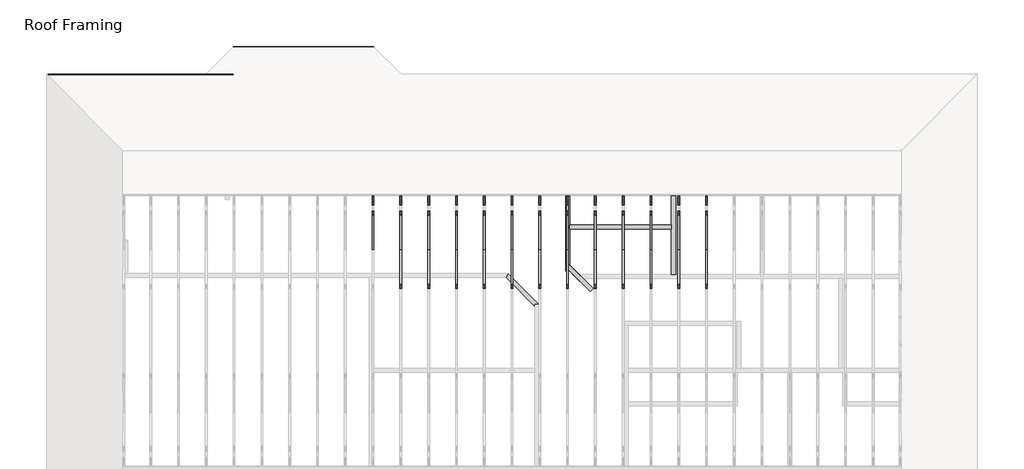
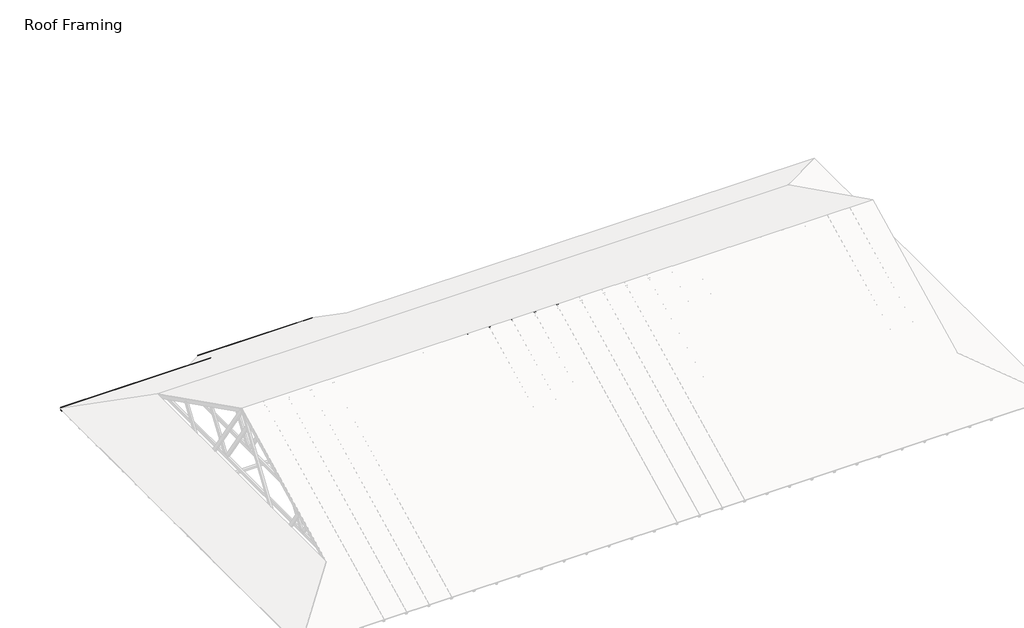
# One storey, part 6 of 7: 43 beams, 25 members.
"""IFC4 building model written with IfcOpenShell, lengths in millimetres."""

import ifcopenshell
import ifcopenshell.guid

model = None  # the IFC model being written
_history = None  # IfcOwnerHistory: only IFC2X3 demands one
_inside = {}  # id of a spatial element -> (the spatial element, [elements in it])
_under = {}  # id of a project, library or spatial element -> (it, [spatial elements below it])
_declared = {}  # id of a project -> (the project, [libraries it declares])
_typed = {}  # id of a type object -> (the type object, [elements of that type])
_made_of = {}  # id of a material, layer set ... -> (it, [elements and type objects made of it])


def new_model(schema):
    """Start an empty IFC model of exactly this schema.

    Asked for "IFC4X3", IfcOpenShell would pick the latest addendum, in which some entities
    have other attributes; the version numbers below select the first issue.
    IFC2X3 requires an IfcOwnerHistory on every rooted entity: one is made here for all.
    """
    global model, _history
    if schema == "IFC4X3":
        model = ifcopenshell.file(schema_version=(4, 3, 0, 0))
    else:
        model = ifcopenshell.file(schema=schema)
    _inside.clear()
    _under.clear()
    _declared.clear()
    _typed.clear()
    _made_of.clear()
    _history = None
    if model.schema == "IFC2X3":
        org = make("IfcOrganization", Name="unknown")
        user = make(
            "IfcPersonAndOrganization",
            ThePerson=make("IfcPerson", FamilyName="unknown"),
            TheOrganization=org,
        )
        app = make(
            "IfcApplication",
            ApplicationDeveloper=org,
            Version="unknown",
            ApplicationFullName="unknown",
            ApplicationIdentifier="unknown",
        )
        _history = make(
            "IfcOwnerHistory",
            OwningUser=user,
            OwningApplication=app,
            ChangeAction="ADDED",
            CreationDate=0,
        )
    return model


def make(cls, **values):
    """One entity of the class cls with the attributes given. An attribute that is None is left unset."""
    return model.create_entity(
        cls, **{name: value for name, value in values.items() if value is not None}
    )


def rooted(cls, **values):
    """An entity with a GlobalId (a new one), such as an element, a storey or a relation."""
    return make(cls, GlobalId=ifcopenshell.guid.new(), OwnerHistory=_history, **values)


def si_unit(unit_type, name, prefix=None):
    """IfcSIUnit, for example si_unit("LENGTHUNIT", "METRE", prefix="MILLI")."""
    return make("IfcSIUnit", UnitType=unit_type, Prefix=prefix, Name=name)


def assignment(units):
    """IfcUnitAssignment: the units of a project."""
    return None if units is None else make("IfcUnitAssignment", Units=units)


def point(xyz):
    """IfcCartesianPoint."""
    return None if xyz is None else make("IfcCartesianPoint", Coordinates=xyz)


def direction(xyz):
    """IfcDirection."""
    return None if xyz is None else make("IfcDirection", DirectionRatios=xyz)


def frame(location, z_axis=None, x_axis=None):
    """IfcAxis2Placement3D, a coordinate frame: its origin and axes. An axis left out is left unset."""
    return make(
        "IfcAxis2Placement3D",
        Location=point(location),
        Axis=direction(z_axis),
        RefDirection=direction(x_axis),
    )


def origin():
    """The frame at (0, 0, 0) with its axes left unset."""
    return frame((0.0, 0.0, 0.0))


def place(relative_to, where):
    """IfcLocalPlacement: puts the frame where relative to a parent placement (None: the world)."""
    return make(
        "IfcLocalPlacement", PlacementRelTo=relative_to, RelativePlacement=where
    )


def context(
    kind, dimensions, precision=None, world=None, true_north=None, identifier=None
):
    """IfcGeometricRepresentationContext, for example the 3D "Model" context."""
    return make(
        "IfcGeometricRepresentationContext",
        ContextIdentifier=identifier,
        ContextType=kind,
        CoordinateSpaceDimension=dimensions,
        Precision=precision,
        WorldCoordinateSystem=world,
        TrueNorth=true_north,
    )


def project(units=None, contexts=None):
    """IfcProject with its units and contexts."""
    return rooted(
        "IfcProject",
        Name="project",
        RepresentationContexts=contexts,
        UnitsInContext=assignment(units),
    )


def spatial(cls, under=None, at=None, **own):
    """A site, building, storey or space (cls), placed at a placement, below another one or the project."""
    s = rooted(cls, ObjectPlacement=at, **own)
    if under is not None:
        _under.setdefault(under.id(), (under, []))[1].append(s)
    return s


def polyline(points):
    """IfcPolyline through the points."""
    return make("IfcPolyline", Points=[point(p) for p in points])


def outline(outer, holes=None, kind="AREA"):
    """IfcArbitraryClosedProfileDef: a profile drawn as a closed curve; with holes, ...WithVoids."""
    if holes is None:
        return make("IfcArbitraryClosedProfileDef", ProfileType=kind, OuterCurve=outer)
    return make(
        "IfcArbitraryProfileDefWithVoids",
        ProfileType=kind,
        OuterCurve=outer,
        InnerCurves=holes,
    )


def extrude(swept, where, along, depth):
    """IfcExtrudedAreaSolid: the profile swept, set in the frame where, extruded along a direction by depth."""
    return make(
        "IfcExtrudedAreaSolid",
        SweptArea=swept,
        Position=where,
        ExtrudedDirection=direction(along),
        Depth=depth,
    )


def faces_of(points, faces, orient=None, outer=None):
    """IfcFace entities. A face is a list of loops; a loop is a list of indices into points, from 0.

    orient and outer hold one flag for each loop. By default every Orientation is true, the
    first loop of a face is its IfcFaceOuterBound and the others are IfcFaceBound.
    """
    made = []
    for i, loops in enumerate(faces):
        bounds = []
        for j, loop in enumerate(loops):
            is_outer = j == 0 if outer is None else outer[i][j]
            bounds.append(
                make(
                    "IfcFaceOuterBound" if is_outer else "IfcFaceBound",
                    Bound=make("IfcPolyLoop", Polygon=[points[k] for k in loop]),
                    Orientation=True if orient is None else orient[i][j],
                )
            )
        made.append(make("IfcFace", Bounds=bounds))
    return made


def faceted_brep(points, faces, orient=None, outer=None, voids=None):
    """IfcFacetedBrep: a solid bounded by flat faces; with voids (closed shells), ...WithVoids."""
    shared = [point(p) for p in points]
    hull = make("IfcClosedShell", CfsFaces=faces_of(shared, faces, orient, outer))
    if voids is None:
        return make("IfcFacetedBrep", Outer=hull)
    return make(
        "IfcFacetedBrepWithVoids",
        Outer=hull,
        Voids=[
            make(cls, CfsFaces=faces_of(shared, fs, o, b)) for cls, fs, o, b in voids
        ],
    )


def shape(context_of_items, identifier, shape_type, items):
    """IfcShapeRepresentation: the items that make up one representation, for example the "Body"."""
    return make(
        "IfcShapeRepresentation",
        ContextOfItems=context_of_items,
        RepresentationIdentifier=identifier,
        RepresentationType=shape_type,
        Items=items,
    )


def source(mapping_origin, context_of_items, identifier, shape_type, items):
    """IfcRepresentationMap: a shape defined once, which mapped items show again and again."""
    return make(
        "IfcRepresentationMap",
        MappingOrigin=mapping_origin,
        MappedRepresentation=shape(context_of_items, identifier, shape_type, items),
    )


def transform(
    local_origin,
    x_axis=None,
    y_axis=None,
    z_axis=None,
    scale=None,
    scale2=None,
    scale3=None,
    uniform=True,
):
    """IfcCartesianTransformationOperator3D, or its non-uniform kind. x_axis, y_axis, z_axis: its Axis1, 2, 3."""
    if uniform:
        return make(
            "IfcCartesianTransformationOperator3D",
            Axis1=direction(x_axis),
            Axis2=direction(y_axis),
            LocalOrigin=point(local_origin),
            Scale=scale,
            Axis3=direction(z_axis),
        )
    return make(
        "IfcCartesianTransformationOperator3DnonUniform",
        Axis1=direction(x_axis),
        Axis2=direction(y_axis),
        LocalOrigin=point(local_origin),
        Scale=scale,
        Axis3=direction(z_axis),
        Scale2=scale2,
        Scale3=scale3,
    )


def mapped(mapping_source, mapping_target):
    """IfcMappedItem: shows the shape of a source again, moved by a transform."""
    return make(
        "IfcMappedItem", MappingSource=mapping_source, MappingTarget=mapping_target
    )


def made_of(thing, what):
    """Note that an element or type object is made of a material, layer set ...; save() writes the relation."""
    if what is not None:
        _made_of.setdefault(what.id(), (what, []))[1].append(thing)
    return thing


def element(
    cls,
    number,
    at=None,
    inside=None,
    cuts=None,
    type_object=None,
    material=None,
    context=None,
    identifier="Body",
    shape_type=None,
    held_by="IfcProductDefinitionShape",
    body=None,
    shapes=None,
    **own,
):
    """One element of the class cls, such as IfcWall. Its Tag is "e" and its number.

    at: its placement. inside: the storey or other place that contains it. cuts: it is an
    opening in that element (IfcRelVoidsElement). A single representation is given by context,
    identifier, shape_type and body (its items); several are given by shapes. held_by: the class
    of the entity that holds the representations. save() writes the other relations.
    """
    e = rooted(cls, Tag="e%d" % number, ObjectPlacement=at, **own)
    if body is not None:
        shapes = [shape(context, identifier, shape_type, body)]
    if shapes is not None:
        e.Representation = make(held_by, Representations=shapes)
    if inside is not None:
        _inside.setdefault(inside.id(), (inside, []))[1].append(e)
    if cuts is not None:
        rooted(
            "IfcRelVoidsElement", RelatingBuildingElement=cuts, RelatedOpeningElement=e
        )
    if type_object is not None:
        _typed.setdefault(type_object.id(), (type_object, []))[1].append(e)
    return made_of(e, material)


def aggregate(whole, parts):
    """IfcRelAggregates: a whole, such as a stair, and the parts it consists of."""
    return rooted("IfcRelAggregates", RelatingObject=whole, RelatedObjects=parts)


def save(model, path):
    """Write the relations noted so far, then the file.

    IfcRelAggregates (storeys below a building ...), IfcRelContainedInSpatialStructure (elements
    in a storey), IfcRelDefinesByType, IfcRelAssociatesMaterial and IfcRelDeclares: one each for
    every whole, place, type object, material and project.
    """
    for whole, parts in _under.values():
        aggregate(whole, parts)
    for where, things in _inside.values():
        rooted(
            "IfcRelContainedInSpatialStructure",
            RelatedElements=things,
            RelatingStructure=where,
        )
    for kind, things in _typed.values():
        rooted("IfcRelDefinesByType", RelatedObjects=things, RelatingType=kind)
    for what, things in _made_of.values():
        rooted("IfcRelAssociatesMaterial", RelatedObjects=things, RelatingMaterial=what)
    for by, libraries in _declared.values():
        rooted("IfcRelDeclares", RelatingContext=by, RelatedDefinitions=libraries)
    model.write(path)


def dimension_lumber_bf031064(model_context):
    return source(origin(), model_context, "Body", "SweptSolid", [
        extrude(outline(polyline([(13801.725, 19.05), (13801.725, -19.05), (-5743.575, -19.05), (-5743.575, 19.05), (13801.725, 19.05)])), frame((0.0, 0.0, -44.45), z_axis=(0.0, 0.0, 1.0), x_axis=(1.0, 0.0, 0.0)), (0.0, 0.0, 1.0), 88.9),
    ])


def dimension_lumber_94c0e0a3(model_context):
    return source(origin(), model_context, "Body", "SweptSolid", [
        extrude(outline(polyline([(1162.05, 44.45), (1162.05, -44.45), (-1073.15, -44.45), (-1073.15, 44.45), (1162.05, 44.45)])), frame((0.0, 0.0, -19.05), z_axis=(0.0, 0.0, 1.0), x_axis=(1.0, 0.0, 0.0)), (0.0, 0.0, 1.0), 38.1),
    ])


def dimension_lumber_901b61d8(model_context):
    return source(origin(), model_context, "Body", "SweptSolid", [
        extrude(outline(polyline([(1117.6, 44.45), (1117.6, -44.45), (-1117.6, -44.45), (-1117.6, 44.45), (1117.6, 44.45)])), frame((0.0, 0.0, -19.05), z_axis=(0.0, 0.0, 1.0), x_axis=(1.0, 0.0, 0.0)), (0.0, 0.0, 1.0), 38.1),
    ])


def dimension_lumber_386be09e(model_context):
    return source(origin(), model_context, "Body", "SweptSolid", [
        extrude(outline(polyline([(1073.15, 44.45), (1073.15, -44.45), (-1073.15, -44.45), (-1073.15, 44.45), (1073.15, 44.45)])), frame((0.0, 0.0, -19.05), z_axis=(0.0, 0.0, 1.0), x_axis=(1.0, 0.0, 0.0)), (0.0, 0.0, 1.0), 38.1),
    ])


def dimension_lumber_2a703131(model_context):
    return source(origin(), model_context, "Body", "SweptSolid", [
        extrude(outline(polyline([(6275.3875, 44.45), (6275.3875, -44.45), (-6338.8875, -44.45), (-6338.8875, 44.45), (6275.3875, 44.45)])), frame((0.0, 0.0, -19.05), z_axis=(0.0, 0.0, 1.0), x_axis=(1.0, 0.0, 0.0)), (0.0, 0.0, 1.0), 38.1),
    ])


model = new_model("IFC4")

# Units and contexts
model_context = context("Model", 3, world=origin())
ifc_project = project(units=[si_unit("LENGTHUNIT", "METRE", prefix="MILLI")], contexts=[model_context])

# Site, building, storey
site = spatial("IfcSite", under=ifc_project)
building = spatial("IfcBuilding", under=site)
storey = spatial("IfcBuildingStorey", under=building, Name="Roof Framing", Elevation=2768.6)

# Beams
placement = place(None, origin())
element("IfcBeam", 1, ObjectType="Dimension Lumber : Top Supporting Lumbers", at=placement, inside=storey, context=model_context, shape_type="SweptSolid", body=[
    extrude(outline(polyline([(466.1639833, 4361.0431112), (-207.4454144, 5034.6525089), (-144.5836215, 5097.5143017), (529.0257761, 4423.904904), (466.1639833, 4361.0431112)])), frame((0.0, 0.0, 2425.7), z_axis=(0.0, 0.0, 1.0), x_axis=(1.0, 0.0, 0.0)), (0.0, 0.0, 1.0), 38.1),
    extrude(outline(polyline([(466.1639833, 4361.0431112), (-181.7263108, 5008.9334053), (-145.3540057, 5096.7439175), (-144.5836215, 5097.5143017), (529.0257761, 4423.904904), (466.1639833, 4361.0431112)])), frame((0.0, 0.0, 2425.7), z_axis=(0.0, 0.0, 1.0), x_axis=(1.0, 0.0, 0.0)), (0.0, 0.0, 1.0), 38.1),
    extrude(outline(polyline([(427.8736892, 4399.3334053), (-181.7263108, 5008.9334053), (-145.3540057, 5096.7439175), (-144.5836215, 5097.5143017), (529.0257761, 4423.904904), (504.4542774, 4399.3334053), (427.8736892, 4399.3334053)])), frame((0.0, 0.0, 2425.7), z_axis=(0.0, 0.0, 1.0), x_axis=(1.0, 0.0, 0.0)), (0.0, 0.0, 1.0), 38.1),
    extrude(outline(polyline([(427.8736892, 4399.3334053), (-181.7263108, 5008.9334053), (-145.3540057, 5096.7439175), (-144.5836215, 5097.5143017), (472.6347749, 4480.2959053), (472.6347749, 4399.3334053), (427.8736892, 4399.3334053)])), frame((0.0, 0.0, 2425.7), z_axis=(0.0, 0.0, 1.0), x_axis=(1.0, 0.0, 0.0)), (0.0, 0.0, 1.0), 38.1),
    extrude(outline(polyline([(427.8736892, 4399.3334053), (-181.7263108, 5008.9334053), (-145.3540057, 5096.7439175), (-144.5836215, 5097.5143017), (464.6972749, 4488.2334053), (464.6972749, 4399.3334053), (427.8736892, 4399.3334053)])), frame((0.0, 0.0, 2425.7), z_axis=(0.0, 0.0, 1.0), x_axis=(1.0, 0.0, 0.0)), (0.0, 0.0, 1.0), 38.1),
])
element("IfcBeam", 2, ObjectType="Dimension Lumber : Top Supporting Lumbers", at=placement, inside=storey, context=model_context, shape_type="SweptSolid", body=[
    extrude(outline(polyline([(-149.1478744, 5102.0785546), (529.0257761, 4423.904904), (466.1639833, 4361.0431112), (-212.0096673, 5039.2167618), (-149.1478744, 5102.0785546)])), frame((0.0, 0.0, 2387.6), z_axis=(0.0, 0.0, 1.0), x_axis=(1.0, 0.0, 0.0)), (0.0, 0.0, 1.0), 38.1),
    extrude(outline(polyline([(-144.9027251, 5097.8334053), (529.0257761, 4423.904904), (466.1639833, 4361.0431112), (-181.7263108, 5008.9334053), (-144.9027251, 5097.8334053)])), frame((0.0, 0.0, 2387.6), z_axis=(0.0, 0.0, 1.0), x_axis=(1.0, 0.0, 0.0)), (0.0, 0.0, 1.0), 38.1),
    extrude(outline(polyline([(-144.9027251, 5097.8334053), (529.0257761, 4423.904904), (504.4542774, 4399.3334053), (427.8736892, 4399.3334053), (-181.7263108, 5008.9334053), (-144.9027251, 5097.8334053)])), frame((0.0, 0.0, 2387.6), z_axis=(0.0, 0.0, 1.0), x_axis=(1.0, 0.0, 0.0)), (0.0, 0.0, 1.0), 38.1),
    extrude(outline(polyline([(-144.9027251, 5097.8334053), (472.6347749, 4480.2959053), (472.6347749, 4399.3334053), (427.8736892, 4399.3334053), (-181.7263108, 5008.9334053), (-144.9027251, 5097.8334053)])), frame((0.0, 0.0, 2387.6), z_axis=(0.0, 0.0, 1.0), x_axis=(1.0, 0.0, 0.0)), (0.0, 0.0, 1.0), 38.1),
    extrude(outline(polyline([(-144.9027251, 5097.8334053), (464.6972749, 4488.2334053), (464.6972749, 4399.3334053), (427.8736892, 4399.3334053), (-181.7263108, 5008.9334053), (-144.9027251, 5097.8334053)])), frame((0.0, 0.0, 2387.6), z_axis=(0.0, 0.0, 1.0), x_axis=(1.0, 0.0, 0.0)), (0.0, 0.0, 1.0), 38.1),
])
element("IfcBeam", 3, ObjectType="Dimension Lumber : Roof Lumbers", at=placement, inside=storey, context=model_context, shape_type="Brep", body=[
    faceted_brep([(-6671.1152251, 4918.4459053, 2653.50625), (-6671.1152251, 4956.5459053, 2653.50625), (-6671.1152251, 4956.5459053, 2564.60625), (-6671.1152251, 4918.4459053, 2564.60625), (-2613.4652251, 4918.4459053, 2653.50625), (-2613.4652251, 4918.4459053, 2564.60625), (-2613.4652251, 4956.5459053, 2564.60625), (-2613.4652251, 4956.5459053, 2653.50625)], [[[0, 1, 2, 3]], [[4, 5, 6, 7]], [[1, 0, 4, 7]], [[2, 1, 7, 6]], [[3, 2, 6, 5]], [[0, 3, 5, 4]]]),
    faceted_brep([(-6671.1152251, 4956.5459053, 2634.3548743), (-6671.1152251, 4956.5459053, 2564.60625), (-6671.1152251, 4918.4459053, 2564.60625), (-6671.1152251, 4918.4459053, 2653.50625), (-2613.4652251, 4956.5459053, 2634.3548743), (-2613.4652251, 4956.5459053, 2564.60625), (-2613.4652251, 4918.4459053, 2564.60625), (-2613.4652251, 4918.4459053, 2653.50625)], [[[0, 1, 2, 3]], [[1, 0, 4, 5]], [[2, 1, 5, 6]], [[3, 2, 6, 7]], [[7, 6, 5, 4]], [[0, 3, 7, 4]]]),
])
element("IfcBeam", 4, ObjectType="Dimension Lumber : Roof Lumbers", at=placement, inside=storey, context=model_context, shape_type="Brep", body=[
    faceted_brep([(-2613.4652251, 5528.0459053, 2348.70625), (-2613.4652251, 5566.1459053, 2348.70625), (-2613.4652251, 5566.1459053, 2259.80625), (-2613.4652251, 5528.0459053, 2259.80625), (472.6347749, 5528.0459053, 2348.70625), (472.6347749, 5528.0459053, 2259.80625), (472.6347749, 5566.1459053, 2259.80625), (472.6347749, 5566.1459053, 2348.70625)], [[[0, 1, 2, 3]], [[4, 5, 6, 7]], [[1, 0, 4, 7]], [[2, 1, 7, 6]], [[3, 2, 6, 5]], [[0, 3, 5, 4]]]),
    faceted_brep([(-2613.4652251, 5566.1459053, 2329.5548743), (-2613.4652251, 5566.1459053, 2259.80625), (-2613.4652251, 5528.0459053, 2259.80625), (-2613.4652251, 5528.0459053, 2348.70625), (472.6347749, 5566.1459053, 2329.5548743), (472.6347749, 5566.1459053, 2259.80625), (472.6347749, 5528.0459053, 2259.80625), (472.6347749, 5528.0459053, 2348.70625)], [[[0, 1, 2, 3]], [[1, 0, 4, 5]], [[2, 1, 5, 6]], [[3, 2, 6, 7]], [[7, 6, 5, 4]], [[0, 3, 7, 4]]]),
])
element("IfcBeam", 5, ObjectType="Dimension Lumber : Roof Lumbers", at=placement, inside=storey, context=model_context, shape_type="SweptSolid", body=[
    extrude(outline(polyline([(-2613.4652251, 5108.9459053), (-2613.4652251, 5147.0459053), (472.6347749, 5147.0459053), (472.6347749, 5108.9459053), (-2613.4652251, 5108.9459053)])), frame((0.0, 0.0, 2259.80625), z_axis=(0.0, 0.0, 1.0), x_axis=(1.0, 0.0, 0.0)), (0.0, 0.0, 1.0), 88.9),
])
element("IfcBeam", 6, ObjectType="Dimension Lumber : Top Supporting Lumbers", at=placement, inside=storey, context=model_context, shape_type="SweptSolid", body=[
    extrude(outline(polyline([(4765.2347749, 638.6232039), (4676.3347749, 638.6232039), (4676.3347749, 4399.3334053), (4765.2347749, 4399.3334053), (4765.2347749, 638.6232039)])), frame((0.0, 0.0, 2692.4), z_axis=(0.0, 0.0, 1.0), x_axis=(1.0, 0.0, 0.0)), (0.0, 0.0, 1.0), 38.1),
    extrude(outline(polyline([(4676.3347749, 727.4459053), (4676.3347749, 4399.3334053), (4765.2347749, 4399.3334053), (4765.2347749, 764.269491), (4676.3347749, 727.4459053)])), frame((0.0, 0.0, 2692.4), z_axis=(0.0, 0.0, 1.0), x_axis=(1.0, 0.0, 0.0)), (0.0, 0.0, 1.0), 38.1),
])
element("IfcBeam", 7, ObjectType="Dimension Lumber : Top Supporting Lumbers", at=placement, inside=storey, context=model_context, shape_type="SweptSolid", body=[
    extrude(outline(polyline([(5056.0583606, 473.4459053), (4993.1965677, 410.5841125), (4676.3347749, 727.4459053), (4765.2347749, 764.269491), (5056.0583606, 473.4459053)])), frame((0.0, 0.0, 2692.4), z_axis=(0.0, 0.0, 1.0), x_axis=(1.0, 0.0, 0.0)), (0.0, 0.0, 1.0), 38.1),
    extrude(outline(polyline([(4930.3347749, 473.4459053), (4676.3347749, 727.4459053), (4765.2347749, 764.269491), (4967.1583606, 562.3459053), (4930.3347749, 473.4459053)])), frame((0.0, 0.0, 2692.4), z_axis=(0.0, 0.0, 1.0), x_axis=(1.0, 0.0, 0.0)), (0.0, 0.0, 1.0), 38.1),
])
element("IfcBeam", 8, ObjectType="Dimension Lumber : Top Supporting Lumbers", at=placement, inside=storey, context=model_context, shape_type="SweptSolid", body=[
    extrude(outline(polyline([(4086.2782231, -98.5475429), (4023.4164303, -161.4093358), (3372.6861892, 489.3209053), (3409.5097749, 578.2209053), (4086.2782231, -98.5475429)])), frame((0.0, 0.0, 2692.4), z_axis=(0.0, 0.0, 1.0), x_axis=(1.0, 0.0, 0.0)), (0.0, 0.0, 1.0), 38.1),
    extrude(outline(polyline([(3996.8847749, -134.8776804), (3372.6861892, 489.3209053), (3409.5097749, 578.2209053), (4085.7847749, -98.0540947), (3996.8847749, -134.8776804)])), frame((0.0, 0.0, 2692.4), z_axis=(0.0, 0.0, 1.0), x_axis=(1.0, 0.0, 0.0)), (0.0, 0.0, 1.0), 38.1),
])
element("IfcBeam", 9, ObjectType="Dimension Lumber : Top Supporting Lumbers", at=placement, inside=storey, context=model_context, shape_type="SweptSolid", body=[
    extrude(outline(polyline([(4676.3347749, 4399.3334053), (4765.2347749, 4399.3334053), (4765.2347749, 764.269491), (4676.3347749, 727.4459053), (4676.3347749, 4399.3334053)])), frame((0.0, 0.0, 2730.5), z_axis=(0.0, 0.0, 1.0), x_axis=(1.0, 0.0, 0.0)), (0.0, 0.0, 1.0), 38.1),
])
element("IfcBeam", 10, ObjectType="Dimension Lumber : Top Supporting Lumbers", at=placement, inside=storey, context=model_context, shape_type="SweptSolid", body=[
    extrude(outline(polyline([(4677.0339804, 726.7466998), (4739.8957732, 789.6084927), (5281.6079113, 247.8963545), (5218.7461185, 185.0345617), (4677.0339804, 726.7466998)])), frame((0.0, 0.0, 2730.5), z_axis=(0.0, 0.0, 1.0), x_axis=(1.0, 0.0, 0.0)), (0.0, 0.0, 1.0), 38.1),
    extrude(outline(polyline([(4677.0339804, 726.7466998), (4678.7220117, 728.4347312), (4765.2347749, 764.269491), (5281.6079113, 247.8963545), (5218.7461185, 185.0345617), (4677.0339804, 726.7466998)])), frame((0.0, 0.0, 2730.5), z_axis=(0.0, 0.0, 1.0), x_axis=(1.0, 0.0, 0.0)), (0.0, 0.0, 1.0), 38.1),
    extrude(outline(polyline([(4677.0339804, 726.7466998), (4678.7220117, 728.4347312), (4765.2347749, 764.269491), (4967.1583606, 562.3459053), (4930.3347749, 473.4459053), (4677.0339804, 726.7466998)])), frame((0.0, 0.0, 2730.5), z_axis=(0.0, 0.0, 1.0), x_axis=(1.0, 0.0, 0.0)), (0.0, 0.0, 1.0), 38.1),
])
dimension_lumber_shape = dimension_lumber_bf031064(model_context)
element("IfcBeam", 11, ObjectType="Dimension Lumber : Roof Lumbers", at=placement, inside=storey, context=model_context, shape_type="MappedRepresentation", body=[
    mapped(dimension_lumber_shape, transform((7511.6097749, 4518.3959053, 2609.05625), x_axis=(-1.0, 0.0, 0.0), y_axis=(0.0, -1.0, 0.0), z_axis=(0.0, 0.0, 1.0))),
])
dimension_lumber_2_shape = dimension_lumber_94c0e0a3(model_context)
element("IfcBeam", 12, ObjectType="Dimension Lumber : Top Supporting Lumbers", at=placement, inside=storey, context=model_context, shape_type="MappedRepresentation", body=[
    mapped(dimension_lumber_2_shape, transform((7044.8847749, 1635.4959053, 2711.45), x_axis=(0.0, 1.0, 0.0), y_axis=(-1.0, 0.0, 0.0), z_axis=(0.0, 0.0, 1.0))),
])
dimension_lumber_3_shape = dimension_lumber_901b61d8(model_context)
element("IfcBeam", 13, ObjectType="Dimension Lumber : Top Supporting Lumbers", at=placement, inside=storey, context=model_context, shape_type="MappedRepresentation", body=[
    mapped(dimension_lumber_3_shape, transform((5882.8347749, 1597.3959053, 2711.45), x_axis=(-1.0, 0.0, 0.0), y_axis=(0.0, -1.0, 0.0), z_axis=(0.0, 0.0, 1.0))),
])
element("IfcBeam", 14, ObjectType="Dimension Lumber : Top Supporting Lumbers", at=placement, inside=storey, context=model_context, shape_type="MappedRepresentation", body=[
    mapped(dimension_lumber_3_shape, transform((5882.8347749, 1597.3959053, 2749.55), x_axis=(1.0, 0.0, 0.0), y_axis=(0.0, 1.0, 0.0), z_axis=(0.0, 0.0, 1.0))),
])
dimension_lumber_4_shape = dimension_lumber_386be09e(model_context)
element("IfcBeam", 15, ObjectType="Dimension Lumber : Top Supporting Lumbers", at=placement, inside=storey, context=model_context, shape_type="MappedRepresentation", body=[
    mapped(dimension_lumber_4_shape, transform((7044.8847749, 1635.4959053, 2749.55), x_axis=(0.0, 1.0, 0.0), y_axis=(-1.0, 0.0, 0.0), z_axis=(0.0, 0.0, 1.0))),
])
dimension_lumber_5_shape = dimension_lumber_2a703131(model_context)
element("IfcBeam", 16, ObjectType="Dimension Lumber : Top Supporting Lumbers", at=placement, inside=storey, context=model_context, shape_type="MappedRepresentation", body=[
    mapped(dimension_lumber_5_shape, transform((6879.7847749, 4443.7834053, 2749.55), x_axis=(1.0, 0.0, 0.0), y_axis=(0.0, 1.0, 0.0), z_axis=(0.0, 0.0, 1.0))),
])
element("IfcBeam", 17, ObjectType="Dimension Lumber : Top Supporting Lumbers", at=placement, inside=storey, context=model_context, shape_type="MappedRepresentation", body=[
    mapped(dimension_lumber_5_shape, transform((6879.7847749, 4443.7834053, 2711.45), x_axis=(1.0, 0.0, 0.0), y_axis=(0.0, 1.0, 0.0), z_axis=(0.0, 0.0, 1.0))),
])
element("IfcBeam", 18, ObjectType="Dimension Lumber : 2x4 Blocking", at=placement, inside=storey, context=model_context, shape_type="SweptSolid", body=[
    extrude(outline(polyline([(7787.8347749, 4918.4459053), (7787.8347749, 4537.4459053), (7749.7347749, 4537.4459053), (7749.7347749, 4918.4459053), (7787.8347749, 4918.4459053)])), frame((0.0, 0.0, 2564.60625), z_axis=(0.0, 0.0, 1.0), x_axis=(1.0, 0.0, 0.0)), (0.0, 0.0, 1.0), 88.9),
    extrude(outline(polyline([(4897.2567107, 2564.60625), (4537.4459053, 2564.60625), (4537.4459053, 2653.50625), (4719.4567107, 2653.50625), (4897.2567107, 2564.60625)])), frame((7749.7347749, 0.0, 0.0), z_axis=(1.0, 0.0, 0.0), x_axis=(0.0, 1.0, 0.0)), (0.0, 0.0, 1.0), 38.1),
])
element("IfcBeam", 19, ObjectType="Dimension Lumber : 2x4 Blocking", at=placement, inside=storey, context=model_context, shape_type="SweptSolid", body=[
    extrude(outline(polyline([(7178.2347749, 4918.4459053), (7178.2347749, 4537.4459053), (7140.1347749, 4537.4459053), (7140.1347749, 4918.4459053), (7178.2347749, 4918.4459053)])), frame((0.0, 0.0, 2564.60625), z_axis=(0.0, 0.0, 1.0), x_axis=(1.0, 0.0, 0.0)), (0.0, 0.0, 1.0), 88.9),
    extrude(outline(polyline([(4897.2567107, 2564.60625), (4537.4459053, 2564.60625), (4537.4459053, 2653.50625), (4719.4567107, 2653.50625), (4897.2567107, 2564.60625)])), frame((7140.1347749, 0.0, 0.0), z_axis=(1.0, 0.0, 0.0), x_axis=(0.0, 1.0, 0.0)), (0.0, 0.0, 1.0), 38.1),
])
element("IfcBeam", 20, ObjectType="Dimension Lumber : 2x4 Blocking", at=placement, inside=storey, context=model_context, shape_type="SweptSolid", body=[
    extrude(outline(polyline([(6568.6347749, 4918.4459053), (6568.6347749, 4537.4459053), (6530.5347749, 4537.4459053), (6530.5347749, 4918.4459053), (6568.6347749, 4918.4459053)])), frame((0.0, 0.0, 2564.60625), z_axis=(0.0, 0.0, 1.0), x_axis=(1.0, 0.0, 0.0)), (0.0, 0.0, 1.0), 88.9),
    extrude(outline(polyline([(4897.2567107, 2564.60625), (4537.4459053, 2564.60625), (4537.4459053, 2653.50625), (4719.4567107, 2653.50625), (4897.2567107, 2564.60625)])), frame((6530.5347749, 0.0, 0.0), z_axis=(1.0, 0.0, 0.0), x_axis=(0.0, 1.0, 0.0)), (0.0, 0.0, 1.0), 38.1),
])
element("IfcBeam", 21, ObjectType="Dimension Lumber : 2x4 Blocking", at=placement, inside=storey, context=model_context, shape_type="SweptSolid", body=[
    extrude(outline(polyline([(5959.0347749, 4918.4459053), (5959.0347749, 4537.4459053), (5920.9347749, 4537.4459053), (5920.9347749, 4918.4459053), (5959.0347749, 4918.4459053)])), frame((0.0, 0.0, 2564.60625), z_axis=(0.0, 0.0, 1.0), x_axis=(1.0, 0.0, 0.0)), (0.0, 0.0, 1.0), 88.9),
    extrude(outline(polyline([(4897.2567107, 2564.60625), (4537.4459053, 2564.60625), (4537.4459053, 2653.50625), (4719.4567107, 2653.50625), (4897.2567107, 2564.60625)])), frame((5920.9347749, 0.0, 0.0), z_axis=(1.0, 0.0, 0.0), x_axis=(0.0, 1.0, 0.0)), (0.0, 0.0, 1.0), 38.1),
])
element("IfcBeam", 22, ObjectType="Dimension Lumber : 2x4 Blocking", at=placement, inside=storey, context=model_context, shape_type="SweptSolid", body=[
    extrude(outline(polyline([(5349.4347749, 4918.4459053), (5349.4347749, 4537.4459053), (5311.3347749, 4537.4459053), (5311.3347749, 4918.4459053), (5349.4347749, 4918.4459053)])), frame((0.0, 0.0, 2564.60625), z_axis=(0.0, 0.0, 1.0), x_axis=(1.0, 0.0, 0.0)), (0.0, 0.0, 1.0), 88.9),
    extrude(outline(polyline([(4897.2567107, 2564.60625), (4537.4459053, 2564.60625), (4537.4459053, 2653.50625), (4719.4567107, 2653.50625), (4897.2567107, 2564.60625)])), frame((5311.3347749, 0.0, 0.0), z_axis=(1.0, 0.0, 0.0), x_axis=(0.0, 1.0, 0.0)), (0.0, 0.0, 1.0), 38.1),
])
element("IfcBeam", 23, ObjectType="Dimension Lumber : 2x4 Blocking", at=placement, inside=storey, context=model_context, shape_type="SweptSolid", body=[
    extrude(outline(polyline([(4739.8347749, 4918.4459053), (4739.8347749, 4537.4459053), (4701.7347749, 4537.4459053), (4701.7347749, 4918.4459053), (4739.8347749, 4918.4459053)])), frame((0.0, 0.0, 2564.60625), z_axis=(0.0, 0.0, 1.0), x_axis=(1.0, 0.0, 0.0)), (0.0, 0.0, 1.0), 88.9),
    extrude(outline(polyline([(4897.2567107, 2564.60625), (4537.4459053, 2564.60625), (4537.4459053, 2653.50625), (4719.4567107, 2653.50625), (4897.2567107, 2564.60625)])), frame((4701.7347749, 0.0, 0.0), z_axis=(1.0, 0.0, 0.0), x_axis=(0.0, 1.0, 0.0)), (0.0, 0.0, 1.0), 38.1),
])
element("IfcBeam", 24, ObjectType="Dimension Lumber : 2x4 Blocking", at=placement, inside=storey, context=model_context, shape_type="SweptSolid", body=[
    extrude(outline(polyline([(4130.2347749, 4918.4459053), (4130.2347749, 4537.4459053), (4092.1347749, 4537.4459053), (4092.1347749, 4918.4459053), (4130.2347749, 4918.4459053)])), frame((0.0, 0.0, 2564.60625), z_axis=(0.0, 0.0, 1.0), x_axis=(1.0, 0.0, 0.0)), (0.0, 0.0, 1.0), 88.9),
    extrude(outline(polyline([(4897.2567107, 2564.60625), (4537.4459053, 2564.60625), (4537.4459053, 2653.50625), (4719.4567107, 2653.50625), (4897.2567107, 2564.60625)])), frame((4092.1347749, 0.0, 0.0), z_axis=(1.0, 0.0, 0.0), x_axis=(0.0, 1.0, 0.0)), (0.0, 0.0, 1.0), 38.1),
])
element("IfcBeam", 25, ObjectType="Dimension Lumber : 2x4 Blocking", at=placement, inside=storey, context=model_context, shape_type="SweptSolid", body=[
    extrude(outline(polyline([(3520.6347749, 4918.4459053), (3520.6347749, 4537.4459053), (3482.5347749, 4537.4459053), (3482.5347749, 4918.4459053), (3520.6347749, 4918.4459053)])), frame((0.0, 0.0, 2564.60625), z_axis=(0.0, 0.0, 1.0), x_axis=(1.0, 0.0, 0.0)), (0.0, 0.0, 1.0), 88.9),
    extrude(outline(polyline([(4897.2567107, 2564.60625), (4537.4459053, 2564.60625), (4537.4459053, 2653.50625), (4719.4567107, 2653.50625), (4897.2567107, 2564.60625)])), frame((3482.5347749, 0.0, 0.0), z_axis=(1.0, 0.0, 0.0), x_axis=(0.0, 1.0, 0.0)), (0.0, 0.0, 1.0), 38.1),
])
element("IfcBeam", 26, ObjectType="Dimension Lumber : 2x4 Blocking", at=placement, inside=storey, context=model_context, shape_type="SweptSolid", body=[
    extrude(outline(polyline([(2911.0347749, 4918.4459053), (2911.0347749, 4537.4459053), (2872.9347749, 4537.4459053), (2872.9347749, 4918.4459053), (2911.0347749, 4918.4459053)])), frame((0.0, 0.0, 2564.60625), z_axis=(0.0, 0.0, 1.0), x_axis=(1.0, 0.0, 0.0)), (0.0, 0.0, 1.0), 88.9),
    extrude(outline(polyline([(4897.2567107, 2564.60625), (4537.4459053, 2564.60625), (4537.4459053, 2653.50625), (4719.4567107, 2653.50625), (4897.2567107, 2564.60625)])), frame((2872.9347749, 0.0, 0.0), z_axis=(1.0, 0.0, 0.0), x_axis=(0.0, 1.0, 0.0)), (0.0, 0.0, 1.0), 38.1),
])
element("IfcBeam", 27, ObjectType="Dimension Lumber : 2x4 Blocking", at=placement, inside=storey, context=model_context, shape_type="SweptSolid", body=[
    extrude(outline(polyline([(434.5347749, 5147.0459053), (434.5347749, 5528.0459053), (472.6347749, 5528.0459053), (472.6347749, 5147.0459053), (434.5347749, 5147.0459053)])), frame((0.0, 0.0, 2259.80625), z_axis=(0.0, 0.0, 1.0), x_axis=(1.0, 0.0, 0.0)), (0.0, 0.0, 1.0), 88.9),
    extrude(outline(polyline([(5147.0459053, 2348.70625), (5329.0567107, 2348.70625), (5506.8567107, 2259.80625), (5147.0459053, 2259.80625), (5147.0459053, 2348.70625)])), frame((434.5347749, 0.0, 0.0), z_axis=(1.0, 0.0, 0.0), x_axis=(0.0, 1.0, 0.0)), (0.0, 0.0, 1.0), 38.1),
])
element("IfcBeam", 28, ObjectType="Dimension Lumber : 2x4 Blocking", at=placement, inside=storey, context=model_context, shape_type="SweptSolid", body=[
    extrude(outline(polyline([(2301.4347749, 4918.4459053), (2301.4347749, 4537.4459053), (2263.3347749, 4537.4459053), (2263.3347749, 4918.4459053), (2301.4347749, 4918.4459053)])), frame((0.0, 0.0, 2564.60625), z_axis=(0.0, 0.0, 1.0), x_axis=(1.0, 0.0, 0.0)), (0.0, 0.0, 1.0), 88.9),
    extrude(outline(polyline([(4897.2567107, 2564.60625), (4537.4459053, 2564.60625), (4537.4459053, 2653.50625), (4719.4567107, 2653.50625), (4897.2567107, 2564.60625)])), frame((2263.3347749, 0.0, 0.0), z_axis=(1.0, 0.0, 0.0), x_axis=(0.0, 1.0, 0.0)), (0.0, 0.0, 1.0), 38.1),
])
element("IfcBeam", 29, ObjectType="Dimension Lumber : 2x4 Blocking", at=placement, inside=storey, context=model_context, shape_type="SweptSolid", body=[
    extrude(outline(polyline([(1653.7347749, 4537.4459053), (1653.7347749, 4918.4459053), (1691.8347749, 4918.4459053), (1691.8347749, 4537.4459053), (1653.7347749, 4537.4459053)])), frame((0.0, 0.0, 2564.60625), z_axis=(0.0, 0.0, 1.0), x_axis=(1.0, 0.0, 0.0)), (0.0, 0.0, 1.0), 88.9),
    extrude(outline(polyline([(4537.4459053, 2653.50625), (4719.4567107, 2653.50625), (4897.2567107, 2564.60625), (4537.4459053, 2564.60625), (4537.4459053, 2653.50625)])), frame((1653.7347749, 0.0, 0.0), z_axis=(1.0, 0.0, 0.0), x_axis=(0.0, 1.0, 0.0)), (0.0, 0.0, 1.0), 38.1),
])
element("IfcBeam", 30, ObjectType="Dimension Lumber : 2x4 Blocking", at=placement, inside=storey, context=model_context, shape_type="SweptSolid", body=[
    extrude(outline(polyline([(1044.1347749, 4537.4459053), (1044.1347749, 4918.4459053), (1082.2347749, 4918.4459053), (1082.2347749, 4537.4459053), (1044.1347749, 4537.4459053)])), frame((0.0, 0.0, 2564.60625), z_axis=(0.0, 0.0, 1.0), x_axis=(1.0, 0.0, 0.0)), (0.0, 0.0, 1.0), 88.9),
    extrude(outline(polyline([(4537.4459053, 2653.50625), (4719.4567107, 2653.50625), (4897.2567107, 2564.60625), (4537.4459053, 2564.60625), (4537.4459053, 2653.50625)])), frame((1044.1347749, 0.0, 0.0), z_axis=(1.0, 0.0, 0.0), x_axis=(0.0, 1.0, 0.0)), (0.0, 0.0, 1.0), 38.1),
])
element("IfcBeam", 31, ObjectType="Dimension Lumber : 2x4 Truss", at=placement, inside=storey, context=model_context, shape_type="SweptSolid", body=[
    extrude(outline(polyline([(4956.5459053, 2634.3548743), (4916.7886167, 2554.840297), (-682.2540947, 5354.3616527), (-682.2540947, 5453.7548743), (4956.5459053, 2634.3548743)])), frame((7749.7347749, 0.0, 0.0), z_axis=(1.0, 0.0, 0.0), x_axis=(0.0, 1.0, 0.0)), (0.0, 0.0, 1.0), 38.1),
])
element("IfcBeam", 32, ObjectType="Dimension Lumber : 2x4 Truss", at=placement, inside=storey, context=model_context, shape_type="SweptSolid", body=[
    extrude(outline(polyline([(4956.5459053, 2634.3548743), (4916.7886167, 2554.840297), (-682.2540947, 5354.3616527), (-682.2540947, 5453.7548743), (4956.5459053, 2634.3548743)])), frame((7140.1347749, 0.0, 0.0), z_axis=(1.0, 0.0, 0.0), x_axis=(0.0, 1.0, 0.0)), (0.0, 0.0, 1.0), 38.1),
])
element("IfcBeam", 33, ObjectType="Dimension Lumber : 2x4 Truss", at=placement, inside=storey, context=model_context, shape_type="SweptSolid", body=[
    extrude(outline(polyline([(4956.5459053, 2634.3548743), (4916.7886167, 2554.840297), (-682.2540947, 5354.3616527), (-682.2540947, 5453.7548743), (4956.5459053, 2634.3548743)])), frame((6530.5347749, 0.0, 0.0), z_axis=(1.0, 0.0, 0.0), x_axis=(0.0, 1.0, 0.0)), (0.0, 0.0, 1.0), 38.1),
])
element("IfcBeam", 34, ObjectType="Dimension Lumber : 2x4 Truss", at=placement, inside=storey, context=model_context, shape_type="SweptSolid", body=[
    extrude(outline(polyline([(4956.5459053, 2634.3548743), (4916.7886167, 2554.840297), (-682.2540947, 5354.3616527), (-682.2540947, 5453.7548743), (4956.5459053, 2634.3548743)])), frame((5920.9347749, 0.0, 0.0), z_axis=(1.0, 0.0, 0.0), x_axis=(0.0, 1.0, 0.0)), (0.0, 0.0, 1.0), 38.1),
])
element("IfcBeam", 35, ObjectType="Dimension Lumber : 2x4 Truss", at=placement, inside=storey, context=model_context, shape_type="SweptSolid", body=[
    extrude(outline(polyline([(4956.5459053, 2634.3548743), (4916.7886167, 2554.840297), (-682.2540947, 5354.3616527), (-682.2540947, 5453.7548743), (4956.5459053, 2634.3548743)])), frame((5311.3347749, 0.0, 0.0), z_axis=(1.0, 0.0, 0.0), x_axis=(0.0, 1.0, 0.0)), (0.0, 0.0, 1.0), 38.1),
])
element("IfcBeam", 36, ObjectType="Dimension Lumber : 2x4 Truss", at=placement, inside=storey, context=model_context, shape_type="SweptSolid", body=[
    extrude(outline(polyline([(4956.5459053, 2634.3548743), (4916.7886167, 2554.840297), (-682.2540947, 5354.3616527), (-682.2540947, 5453.7548743), (4956.5459053, 2634.3548743)])), frame((4701.7347749, 0.0, 0.0), z_axis=(1.0, 0.0, 0.0), x_axis=(0.0, 1.0, 0.0)), (0.0, 0.0, 1.0), 38.1),
])
element("IfcBeam", 37, ObjectType="Dimension Lumber : 2x4 Truss", at=placement, inside=storey, context=model_context, shape_type="SweptSolid", body=[
    extrude(outline(polyline([(4956.5459053, 2634.3548743), (4916.7886167, 2554.840297), (-682.2540947, 5354.3616527), (-682.2540947, 5453.7548743), (4956.5459053, 2634.3548743)])), frame((4092.1347749, 0.0, 0.0), z_axis=(1.0, 0.0, 0.0), x_axis=(0.0, 1.0, 0.0)), (0.0, 0.0, 1.0), 38.1),
])
element("IfcBeam", 38, ObjectType="Dimension Lumber : 2x4 Truss", at=placement, inside=storey, context=model_context, shape_type="SweptSolid", body=[
    extrude(outline(polyline([(4956.5459053, 2634.3548743), (4916.7886167, 2554.840297), (-682.2540947, 5354.3616527), (-682.2540947, 5453.7548743), (4956.5459053, 2634.3548743)])), frame((3482.5347749, 0.0, 0.0), z_axis=(1.0, 0.0, 0.0), x_axis=(0.0, 1.0, 0.0)), (0.0, 0.0, 1.0), 38.1),
])
element("IfcBeam", 39, ObjectType="Dimension Lumber : 2x4 Truss", at=placement, inside=storey, context=model_context, shape_type="SweptSolid", body=[
    extrude(outline(polyline([(4956.5459053, 2634.3548743), (4916.7886167, 2554.840297), (-682.2540947, 5354.3616527), (-682.2540947, 5453.7548743), (4956.5459053, 2634.3548743)])), frame((2872.9347749, 0.0, 0.0), z_axis=(1.0, 0.0, 0.0), x_axis=(0.0, 1.0, 0.0)), (0.0, 0.0, 1.0), 38.1),
])
element("IfcBeam", 40, ObjectType="Dimension Lumber : 2x4 Truss", at=placement, inside=storey, context=model_context, shape_type="SweptSolid", body=[
    extrude(outline(polyline([(4956.5459053, 2634.3548743), (4916.7886167, 2554.840297), (-682.2540947, 5354.3616527), (-682.2540947, 5453.7548743), (4956.5459053, 2634.3548743)])), frame((2263.3347749, 0.0, 0.0), z_axis=(1.0, 0.0, 0.0), x_axis=(0.0, 1.0, 0.0)), (0.0, 0.0, 1.0), 38.1),
])
element("IfcBeam", 41, ObjectType="Dimension Lumber : 2x4 Truss", at=placement, inside=storey, context=model_context, shape_type="SweptSolid", body=[
    extrude(outline(polyline([(4956.5459053, 2634.3548743), (4916.7886167, 2554.840297), (-682.2540947, 5354.3616527), (-682.2540947, 5453.7548743), (4956.5459053, 2634.3548743)])), frame((1653.7347749, 0.0, 0.0), z_axis=(1.0, 0.0, 0.0), x_axis=(0.0, 1.0, 0.0)), (0.0, 0.0, 1.0), 38.1),
])
element("IfcBeam", 42, ObjectType="Dimension Lumber : 2x4 Truss", at=placement, inside=storey, context=model_context, shape_type="SweptSolid", body=[
    extrude(outline(polyline([(4956.5459053, 2634.3548743), (4916.7886167, 2554.840297), (-682.2540947, 5354.3616527), (-682.2540947, 5453.7548743), (4956.5459053, 2634.3548743)])), frame((1044.1347749, 0.0, 0.0), z_axis=(1.0, 0.0, 0.0), x_axis=(0.0, 1.0, 0.0)), (0.0, 0.0, 1.0), 38.1),
])
element("IfcBeam", 43, ObjectType="Dimension Lumber : 2x4 Truss", at=placement, inside=storey, context=model_context, shape_type="SweptSolid", body=[
    extrude(outline(polyline([(4956.5459053, 2634.3548743), (4916.7886167, 2554.840297), (-682.2540947, 5354.3616527), (-682.2540947, 5453.7548743), (4956.5459053, 2634.3548743)])), frame((434.5347749, 0.0, 0.0), z_axis=(1.0, 0.0, 0.0), x_axis=(0.0, 1.0, 0.0)), (0.0, 0.0, 1.0), 38.1),
])

# Members
element("IfcMember", 44, ObjectType="Dimension Lumber : 2x4 Truss", at=placement, inside=storey, context=model_context, shape_type="SweptSolid", body=[
    extrude(outline(polyline([(44.45, 19.05), (44.45, -19.05), (-44.45, -19.05), (-44.45, 19.05), (44.45, 19.05)])), frame((7768.7847749, 1065.7520094, 2831.7897682), z_axis=(0.0, -0.5576002360134061, 0.8301096173384536), x_axis=(0.0, 0.8301096173384536, 0.5576002360134061)), (0.0, 0.0, 1.0), 3068.6997979),
])
element("IfcMember", 45, ObjectType="Dimension Lumber : 2x4 Truss", at=placement, inside=storey, context=model_context, shape_type="SweptSolid", body=[
    extrude(outline(polyline([(44.45, -19.05), (-44.45, -19.05), (-44.45, 19.05), (44.45, 19.05), (44.45, -19.05)])), frame((7768.7847749, 1139.5544724, 2831.7982808), z_axis=(0.0, 0.5576002360134061, 0.8301096173384536), x_axis=(0.0, -0.8301096173384536, 0.5576002360134061)), (0.0, 0.0, 1.0), 1484.7518184),
])
element("IfcMember", 46, ObjectType="Dimension Lumber : 2x4 Truss", at=placement, inside=storey, context=model_context, shape_type="SweptSolid", body=[
    extrude(outline(polyline([(44.45, 19.05), (44.45, -19.05), (-44.45, -19.05), (-44.45, 19.05), (44.45, 19.05)])), frame((7159.1847749, 1065.7520094, 2831.7897682), z_axis=(0.0, -0.5576002360134061, 0.8301096173384536), x_axis=(0.0, 0.8301096173384536, 0.5576002360134061)), (0.0, 0.0, 1.0), 3068.6997979),
])
element("IfcMember", 47, ObjectType="Dimension Lumber : 2x4 Truss", at=placement, inside=storey, context=model_context, shape_type="SweptSolid", body=[
    extrude(outline(polyline([(44.45, -19.05), (-44.45, -19.05), (-44.45, 19.05), (44.45, 19.05), (44.45, -19.05)])), frame((7159.1847749, 1139.5544724, 2831.7982808), z_axis=(0.0, 0.5576002360134061, 0.8301096173384536), x_axis=(0.0, -0.8301096173384536, 0.5576002360134061)), (0.0, 0.0, 1.0), 1484.7518184),
])
element("IfcMember", 48, ObjectType="Dimension Lumber : 2x4 Truss", at=placement, inside=storey, context=model_context, shape_type="SweptSolid", body=[
    extrude(outline(polyline([(44.45, 19.05), (44.45, -19.05), (-44.45, -19.05), (-44.45, 19.05), (44.45, 19.05)])), frame((6549.5847749, 1065.7520094, 2831.7897682), z_axis=(0.0, -0.5576002360134061, 0.8301096173384536), x_axis=(0.0, 0.8301096173384536, 0.5576002360134061)), (0.0, 0.0, 1.0), 3068.6997979),
])
element("IfcMember", 49, ObjectType="Dimension Lumber : 2x4 Truss", at=placement, inside=storey, context=model_context, shape_type="SweptSolid", body=[
    extrude(outline(polyline([(44.45, -19.05), (-44.45, -19.05), (-44.45, 19.05), (44.45, 19.05), (44.45, -19.05)])), frame((6549.5847749, 1139.5544724, 2831.7982808), z_axis=(0.0, 0.5576002360134061, 0.8301096173384536), x_axis=(0.0, -0.8301096173384536, 0.5576002360134061)), (0.0, 0.0, 1.0), 1484.7518184),
])
element("IfcMember", 50, ObjectType="Dimension Lumber : 2x4 Truss", at=placement, inside=storey, context=model_context, shape_type="SweptSolid", body=[
    extrude(outline(polyline([(44.45, 19.05), (44.45, -19.05), (-44.45, -19.05), (-44.45, 19.05), (44.45, 19.05)])), frame((5939.9847749, 1065.7520094, 2831.7897682), z_axis=(0.0, -0.5576002360134061, 0.8301096173384536), x_axis=(0.0, 0.8301096173384536, 0.5576002360134061)), (0.0, 0.0, 1.0), 3068.6997979),
])
element("IfcMember", 51, ObjectType="Dimension Lumber : 2x4 Truss", at=placement, inside=storey, context=model_context, shape_type="SweptSolid", body=[
    extrude(outline(polyline([(44.45, -19.05), (-44.45, -19.05), (-44.45, 19.05), (44.45, 19.05), (44.45, -19.05)])), frame((5939.9847749, 1139.5544724, 2831.7982808), z_axis=(0.0, 0.5576002360134061, 0.8301096173384536), x_axis=(0.0, -0.8301096173384536, 0.5576002360134061)), (0.0, 0.0, 1.0), 1484.7518184),
])
element("IfcMember", 52, ObjectType="Dimension Lumber : 2x4 Truss", at=placement, inside=storey, context=model_context, shape_type="SweptSolid", body=[
    extrude(outline(polyline([(44.45, 19.05), (44.45, -19.05), (-44.45, -19.05), (-44.45, 19.05), (44.45, 19.05)])), frame((5330.3847749, 1065.7520094, 2831.7897682), z_axis=(0.0, -0.5576002360134061, 0.8301096173384536), x_axis=(0.0, 0.8301096173384536, 0.5576002360134061)), (0.0, 0.0, 1.0), 3068.6997979),
])
element("IfcMember", 53, ObjectType="Dimension Lumber : 2x4 Truss", at=placement, inside=storey, context=model_context, shape_type="SweptSolid", body=[
    extrude(outline(polyline([(44.45, -19.05), (-44.45, -19.05), (-44.45, 19.05), (44.45, 19.05), (44.45, -19.05)])), frame((5330.3847749, 1139.5544724, 2831.7982808), z_axis=(0.0, 0.5576002360134061, 0.8301096173384536), x_axis=(0.0, -0.8301096173384536, 0.5576002360134061)), (0.0, 0.0, 1.0), 1484.7518184),
])
element("IfcMember", 54, ObjectType="Dimension Lumber : 2x4 Truss", at=placement, inside=storey, context=model_context, shape_type="SweptSolid", body=[
    extrude(outline(polyline([(44.45, 19.05), (44.45, -19.05), (-44.45, -19.05), (-44.45, 19.05), (44.45, 19.05)])), frame((4720.7847749, 1065.7520094, 2831.7897682), z_axis=(0.0, -0.5576002360134061, 0.8301096173384536), x_axis=(0.0, 0.8301096173384536, 0.5576002360134061)), (0.0, 0.0, 1.0), 3068.6997979),
])
element("IfcMember", 55, ObjectType="Dimension Lumber : 2x4 Truss", at=placement, inside=storey, context=model_context, shape_type="SweptSolid", body=[
    extrude(outline(polyline([(44.45, -19.05), (-44.45, -19.05), (-44.45, 19.05), (44.45, 19.05), (44.45, -19.05)])), frame((4720.7847749, 1139.5544724, 2831.7982808), z_axis=(0.0, 0.5576002360134061, 0.8301096173384536), x_axis=(0.0, -0.8301096173384536, 0.5576002360134061)), (0.0, 0.0, 1.0), 1484.7518184),
])
element("IfcMember", 56, ObjectType="Dimension Lumber : 2x4 Truss", at=placement, inside=storey, context=model_context, shape_type="SweptSolid", body=[
    extrude(outline(polyline([(44.45, 19.05), (44.45, -19.05), (-44.45, -19.05), (-44.45, 19.05), (44.45, 19.05)])), frame((4111.1847749, 1065.7520094, 2831.7897682), z_axis=(0.0, -0.5576002360134061, 0.8301096173384536), x_axis=(0.0, 0.8301096173384536, 0.5576002360134061)), (0.0, 0.0, 1.0), 3068.6997979),
])
element("IfcMember", 57, ObjectType="Dimension Lumber : 2x4 Truss", at=placement, inside=storey, context=model_context, shape_type="SweptSolid", body=[
    extrude(outline(polyline([(44.45, -19.05), (-44.45, -19.05), (-44.45, 19.05), (44.45, 19.05), (44.45, -19.05)])), frame((4111.1847749, 1139.5544724, 2831.7982808), z_axis=(0.0, 0.5576002360134061, 0.8301096173384536), x_axis=(0.0, -0.8301096173384536, 0.5576002360134061)), (0.0, 0.0, 1.0), 1484.7518184),
])
element("IfcMember", 58, ObjectType="Dimension Lumber : 2x4 Truss", at=placement, inside=storey, context=model_context, shape_type="SweptSolid", body=[
    extrude(outline(polyline([(44.45, 19.05), (44.45, -19.05), (-44.45, -19.05), (-44.45, 19.05), (44.45, 19.05)])), frame((3501.5847749, 1065.7520094, 2831.7897682), z_axis=(0.0, -0.5576002360134061, 0.8301096173384536), x_axis=(0.0, 0.8301096173384536, 0.5576002360134061)), (0.0, 0.0, 1.0), 3068.6997979),
])
element("IfcMember", 59, ObjectType="Dimension Lumber : 2x4 Truss", at=placement, inside=storey, context=model_context, shape_type="SweptSolid", body=[
    extrude(outline(polyline([(44.45, -19.05), (-44.45, -19.05), (-44.45, 19.05), (44.45, 19.05), (44.45, -19.05)])), frame((3501.5847749, 1139.5544724, 2831.7982808), z_axis=(0.0, 0.5576002360134061, 0.8301096173384536), x_axis=(0.0, -0.8301096173384536, 0.5576002360134061)), (0.0, 0.0, 1.0), 1484.7518184),
])
element("IfcMember", 60, ObjectType="Dimension Lumber : 2x4 Truss", at=placement, inside=storey, context=model_context, shape_type="SweptSolid", body=[
    extrude(outline(polyline([(44.45, 19.05), (44.45, -19.05), (-44.45, -19.05), (-44.45, 19.05), (44.45, 19.05)])), frame((2891.9847749, 1065.7520094, 2831.7897682), z_axis=(0.0, -0.5576002360134061, 0.8301096173384536), x_axis=(0.0, 0.8301096173384536, 0.5576002360134061)), (0.0, 0.0, 1.0), 3068.6997979),
])
element("IfcMember", 61, ObjectType="Dimension Lumber : 2x4 Truss", at=placement, inside=storey, context=model_context, shape_type="SweptSolid", body=[
    extrude(outline(polyline([(44.45, -19.05), (-44.45, -19.05), (-44.45, 19.05), (44.45, 19.05), (44.45, -19.05)])), frame((2891.9847749, 1139.5544724, 2831.7982808), z_axis=(0.0, 0.5576002360134061, 0.8301096173384536), x_axis=(0.0, -0.8301096173384536, 0.5576002360134061)), (0.0, 0.0, 1.0), 1484.7518184),
])
element("IfcMember", 62, ObjectType="Dimension Lumber : 2x4 Truss", at=placement, inside=storey, context=model_context, shape_type="SweptSolid", body=[
    extrude(outline(polyline([(44.45, 19.05), (44.45, -19.05), (-44.45, -19.05), (-44.45, 19.05), (44.45, 19.05)])), frame((2282.3847749, 1065.7520094, 2831.7897682), z_axis=(0.0, -0.5576002360134061, 0.8301096173384536), x_axis=(0.0, 0.8301096173384536, 0.5576002360134061)), (0.0, 0.0, 1.0), 3068.6997979),
])
element("IfcMember", 63, ObjectType="Dimension Lumber : 2x4 Truss", at=placement, inside=storey, context=model_context, shape_type="SweptSolid", body=[
    extrude(outline(polyline([(44.45, -19.05), (-44.45, -19.05), (-44.45, 19.05), (44.45, 19.05), (44.45, -19.05)])), frame((2282.3847749, 1139.5544724, 2831.7982808), z_axis=(0.0, 0.5576002360134061, 0.8301096173384536), x_axis=(0.0, -0.8301096173384536, 0.5576002360134061)), (0.0, 0.0, 1.0), 1484.7518184),
])
element("IfcMember", 64, ObjectType="Dimension Lumber : 2x4 Truss", at=placement, inside=storey, context=model_context, shape_type="SweptSolid", body=[
    extrude(outline(polyline([(44.45, 19.05), (44.45, -19.05), (-44.45, -19.05), (-44.45, 19.05), (44.45, 19.05)])), frame((1672.7847749, 1065.7520094, 2831.7897682), z_axis=(0.0, -0.5576002360134061, 0.8301096173384536), x_axis=(0.0, 0.8301096173384536, 0.5576002360134061)), (0.0, 0.0, 1.0), 3068.6997979),
])
element("IfcMember", 65, ObjectType="Dimension Lumber : 2x4 Truss", at=placement, inside=storey, context=model_context, shape_type="SweptSolid", body=[
    extrude(outline(polyline([(44.45, -19.05), (-44.45, -19.05), (-44.45, 19.05), (44.45, 19.05), (44.45, -19.05)])), frame((1672.7847749, 1139.5544724, 2831.7982808), z_axis=(0.0, 0.5576002360134061, 0.8301096173384536), x_axis=(0.0, -0.8301096173384536, 0.5576002360134061)), (0.0, 0.0, 1.0), 1484.7518184),
])
element("IfcMember", 66, ObjectType="Dimension Lumber : 2x4 Truss", at=placement, inside=storey, context=model_context, shape_type="SweptSolid", body=[
    extrude(outline(polyline([(44.45, 19.05), (44.45, -19.05), (-44.45, -19.05), (-44.45, 19.05), (44.45, 19.05)])), frame((1063.1847749, 1065.7520094, 2831.7897682), z_axis=(0.0, -0.5576002360134061, 0.8301096173384536), x_axis=(0.0, 0.8301096173384536, 0.5576002360134061)), (0.0, 0.0, 1.0), 3068.6997979),
])
element("IfcMember", 67, ObjectType="Dimension Lumber : 2x4 Truss", at=placement, inside=storey, context=model_context, shape_type="SweptSolid", body=[
    extrude(outline(polyline([(44.45, -19.05), (-44.45, -19.05), (-44.45, 19.05), (44.45, 19.05), (44.45, -19.05)])), frame((1063.1847749, 1139.5544724, 2831.7982808), z_axis=(0.0, 0.5576002360134061, 0.8301096173384536), x_axis=(0.0, -0.8301096173384536, 0.5576002360134061)), (0.0, 0.0, 1.0), 1484.7518184),
])
element("IfcMember", 68, ObjectType="Dimension Lumber : 2x4 Truss", at=placement, inside=storey, context=model_context, shape_type="SweptSolid", body=[
    extrude(outline(polyline([(44.45, -19.05), (-44.45, -19.05), (-44.45, 19.05), (44.45, 19.05), (44.45, -19.05)])), frame((453.5847749, 1139.5544724, 2831.7982808), z_axis=(0.0, 0.5576002360134061, 0.8301096173384536), x_axis=(0.0, -0.8301096173384536, 0.5576002360134061)), (0.0, 0.0, 1.0), 1484.7518184),
])

save(model, "model.ifc")

# Revit data of these elements
# Type "Dimension Lumber : Top Supporting Lumbers"
#   Assembly Code = "B10"
#   A = 0.0364583 SF
#   Length [instance default] = 5' - 0"
#   b = 0' - 3 1/2"
#   d = 0' - 1 1/2"
#   Structural Material [instance default] = Softwood, Lumber
# Type "Dimension Lumber : Roof Lumbers"
#   Assembly Code = "B10"
#   A = 0.0364583 SF
#   Length [instance default] = 5' - 0"
#   b = 0' - 1 1/2"
#   d = 0' - 3 1/2"
#   Structural Material [instance default] = Softwood, Lumber
# Type "Dimension Lumber : 2x4 Blocking"
#   Assembly Code = "B10"
#   Cost = 0
#   A = 0.0364583 SF
#   Length [instance default] = 5' - 0"
#   b = 0' - 1 1/2"
#   d = 0' - 3 1/2"
#   Structural Material [instance default] = Softwood, Lumber
# Type "Dimension Lumber : 2x4 Truss"
#   Assembly Code = "B10"
#   Cost = 750
#   A = 0.0364583 SF
#   Length [instance default] = 5' - 0"
#   b = 0' - 1 1/2"
#   d = 0' - 3 1/2"
#   Structural Material [instance default] = Softwood, Lumber
# Elements 1, 2, 6, 7, 8, 9, 10, 12, 13, 14, 15 (IfcBeam, "Dimension Lumber : Top Supporting Lumbers")
#   Structural Material = Douglas Fir #2
#   Phase Created = New Construction
#   Materials on its faces: "Douglas Fir #2"
# Elements 3, 4, 5, 11 (IfcBeam, "Dimension Lumber : Roof Lumbers")
#   Structural Material = Douglas Fir #2
#   Phase Created = New Construction
#   Materials on its faces: "Douglas Fir #2"
# Elements 16, 17 (IfcBeam, "Dimension Lumber : Top Supporting Lumbers")
#   Comments = ""
#   Structural Material = Douglas Fir #2
#   Phase Created = New Construction
#   Materials on its faces: "Douglas Fir #2"
# Elements 18, 19, 20, 21, 22, 23, 24, 25, 26, 27, 28, 29, 30 (IfcBeam, "Dimension Lumber : 2x4 Blocking")
#   Comments = ""
#   Structural Material = Douglas Fir #2
#   Phase Created = New Construction
#   Materials on its faces: "Douglas Fir #2"
# Elements 31, 32, 33, 34, 35, 36, 37, 38, 39, 40, 41, 42, 43 (IfcBeam, "Dimension Lumber : 2x4 Truss")
#   Structural Material = Douglas Fir #2
#   Phase Created = New Construction
#   Materials on its faces: "Douglas Fir #2"
# Elements 44, 45, 46, 47, 48, 49, 50, 51, 52, 53, 54, 55, 56, 57, 58, 59, 60, 61, 62, 63, 64, 65, 66, 67, 68 (IfcMember, "Dimension Lumber : 2x4 Truss")
#   Comments = ""
#   Structural Material = Douglas Fir #2
#   Phase Created = New Construction
#   Materials on its faces: "Douglas Fir #2"
# Materials
#   "Softwood, Lumber": class "Wood", colour RGB 223 192 134, transparency 0, Description = "Pinus Echinata", Cost = 0
#   "Douglas Fir #2": class "Wood", colour RGB 223 192 134, transparency 0, Description = "Pinus Echinata", Cost = 0
